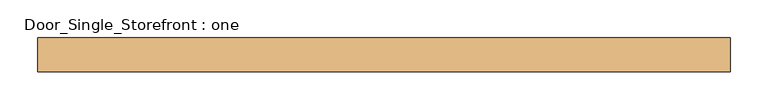
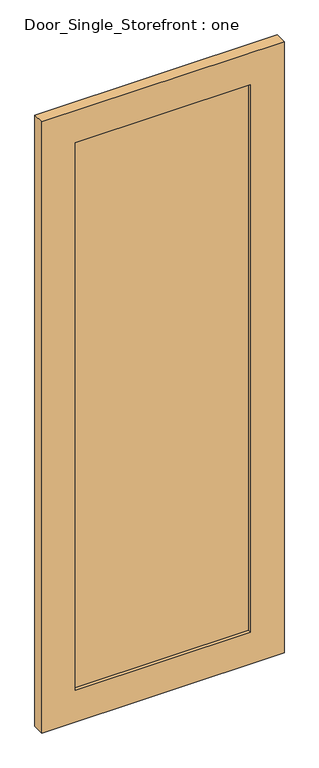
"""IFC4 building model written with IfcOpenShell, lengths in millimetres: door geometry, Door_Single_Storefront : one."""

from ifc_helpers import new_model, si_unit, frame, origin, place, context, project, spatial, polyline, outline, extrude, source, transform, mapped, element, save


def door_single_storefront_one_c51172e4(model_context):
    return source(origin(), model_context, "Body", "SweptSolid", [
        extrude(outline(polyline([(330.2, -6.35), (-330.2, -6.35), (-330.2, 12.7), (330.2, 12.7), (330.2, -6.35)])), frame((0.0, 0.0, 127.0), z_axis=(0.0, 0.0, 1.0), x_axis=(1.0, 0.0, 0.0)), (0.0, 0.0, 1.0), 2184.4),
        extrude(outline(polyline([(2438.4, -457.2), (0.0, -457.2), (0.0, 457.2), (2438.4, 457.2), (2438.4, -457.2)]), holes=[polyline([(127.0, 330.2), (127.0, -330.2), (2311.4, -330.2), (2311.4, 330.2), (127.0, 330.2)])]), frame((0.0, -19.05, 0.0), z_axis=(0.0, 1.0, 0.0), x_axis=(0.0, 0.0, 1.0)), (0.0, 0.0, 1.0), 44.45),
    ])


if __name__ == "__main__":
    model = new_model("IFC4")
    model_context = context("Model", 3, world=origin())
    ifc_project = project(units=[si_unit("LENGTHUNIT", "METRE", prefix="MILLI")], contexts=[model_context])
    site = spatial("IfcSite", under=ifc_project)
    building = spatial("IfcBuilding", under=site)
    placement = place(None, origin())
    door_single_storefront_one_shape = door_single_storefront_one_c51172e4(model_context)
    element("IfcDoor", 1, ObjectType="Door_Single_Storefront : one", at=placement, inside=building, context=model_context, shape_type="MappedRepresentation", body=[
        mapped(door_single_storefront_one_shape, transform((0.0, 0.0, 0.0), x_axis=(1.0, 0.0, 0.0), y_axis=(0.0, 1.0, 0.0), z_axis=(0.0, 0.0, 1.0))),
    ])
    save(model, "model.ifc")

# Revit data of these elements
# Type "Door_Single_Storefront : one"
#   Type Mark = "27"
#   Analytic Construction = "<None>"
#   Stile_Width = 0' - 5"
#   Door_Thickness = 0' - 1 3/4"
#   Door_Offset = 0' - 1"
#   Glass_Material = SAFETY GLAZING
#   Frame_Material = INTERIOR GRADE ALUMINUM STOREFRONT W/ SAFETY GLAZING
#   Function = (empty or 0)
# Element 1 (IfcDoor, "Door_Single_Storefront : one")
#   Materials on its faces: "INTERIOR GRADE ALUMINUM STOREFRONT W/ SAFETY GLAZING", "SAFETY GLAZING"
# Materials
#   "SAFETY GLAZING": class "Glass", colour RGB 142 168 196, transparency 0.75, Description = "Soda Lime Glass", Cost = 0
#   "INTERIOR GRADE ALUMINUM STOREFRONT W/ SAFETY GLAZING": class "Metal", colour RGB 226 226 226, transparency 0, Description = "Aluminum 6061", Cost = 0
